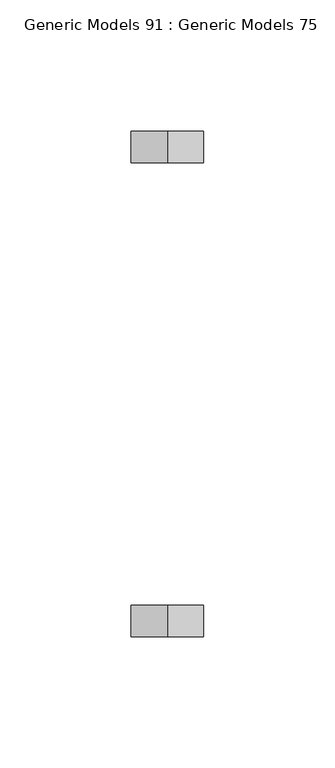
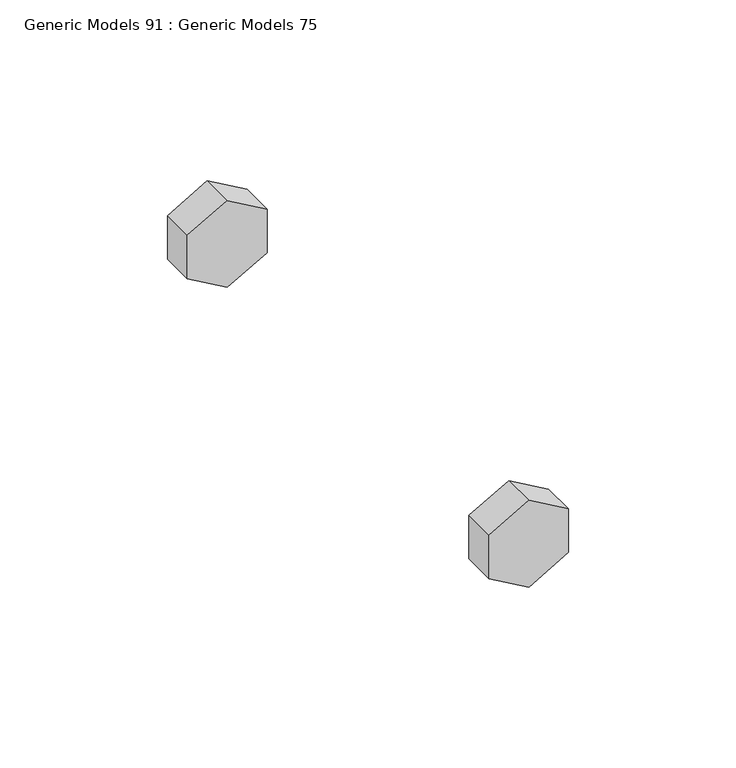
"""IFC4 building model written with IfcOpenShell, lengths in millimetres: proxy geometry, Generic Models 91 : Generic Models 75."""

import ifcopenshell
import ifcopenshell.guid

model = None  # the IFC model being written
_history = None  # IfcOwnerHistory: only IFC2X3 demands one
_inside = {}  # id of a spatial element -> (the spatial element, [elements in it])
_under = {}  # id of a project, library or spatial element -> (it, [spatial elements below it])
_declared = {}  # id of a project -> (the project, [libraries it declares])
_typed = {}  # id of a type object -> (the type object, [elements of that type])
_made_of = {}  # id of a material, layer set ... -> (it, [elements and type objects made of it])


def new_model(schema):
    """Start an empty IFC model of exactly this schema.

    Asked for "IFC4X3", IfcOpenShell would pick the latest addendum, in which some entities
    have other attributes; the version numbers below select the first issue.
    IFC2X3 requires an IfcOwnerHistory on every rooted entity: one is made here for all.
    """
    global model, _history
    if schema == "IFC4X3":
        model = ifcopenshell.file(schema_version=(4, 3, 0, 0))
    else:
        model = ifcopenshell.file(schema=schema)
    _inside.clear()
    _under.clear()
    _declared.clear()
    _typed.clear()
    _made_of.clear()
    _history = None
    if model.schema == "IFC2X3":
        org = make("IfcOrganization", Name="unknown")
        user = make(
            "IfcPersonAndOrganization",
            ThePerson=make("IfcPerson", FamilyName="unknown"),
            TheOrganization=org,
        )
        app = make(
            "IfcApplication",
            ApplicationDeveloper=org,
            Version="unknown",
            ApplicationFullName="unknown",
            ApplicationIdentifier="unknown",
        )
        _history = make(
            "IfcOwnerHistory",
            OwningUser=user,
            OwningApplication=app,
            ChangeAction="ADDED",
            CreationDate=0,
        )
    return model


def make(cls, **values):
    """One entity of the class cls with the attributes given. An attribute that is None is left unset."""
    return model.create_entity(
        cls, **{name: value for name, value in values.items() if value is not None}
    )


def rooted(cls, **values):
    """An entity with a GlobalId (a new one), such as an element, a storey or a relation."""
    return make(cls, GlobalId=ifcopenshell.guid.new(), OwnerHistory=_history, **values)


def si_unit(unit_type, name, prefix=None):
    """IfcSIUnit, for example si_unit("LENGTHUNIT", "METRE", prefix="MILLI")."""
    return make("IfcSIUnit", UnitType=unit_type, Prefix=prefix, Name=name)


def assignment(units):
    """IfcUnitAssignment: the units of a project."""
    return None if units is None else make("IfcUnitAssignment", Units=units)


def point(xyz):
    """IfcCartesianPoint."""
    return None if xyz is None else make("IfcCartesianPoint", Coordinates=xyz)


def direction(xyz):
    """IfcDirection."""
    return None if xyz is None else make("IfcDirection", DirectionRatios=xyz)


def frame(location, z_axis=None, x_axis=None):
    """IfcAxis2Placement3D, a coordinate frame: its origin and axes. An axis left out is left unset."""
    return make(
        "IfcAxis2Placement3D",
        Location=point(location),
        Axis=direction(z_axis),
        RefDirection=direction(x_axis),
    )


def origin():
    """The frame at (0, 0, 0) with its axes left unset."""
    return frame((0.0, 0.0, 0.0))


def place(relative_to, where):
    """IfcLocalPlacement: puts the frame where relative to a parent placement (None: the world)."""
    return make(
        "IfcLocalPlacement", PlacementRelTo=relative_to, RelativePlacement=where
    )


def context(
    kind, dimensions, precision=None, world=None, true_north=None, identifier=None
):
    """IfcGeometricRepresentationContext, for example the 3D "Model" context."""
    return make(
        "IfcGeometricRepresentationContext",
        ContextIdentifier=identifier,
        ContextType=kind,
        CoordinateSpaceDimension=dimensions,
        Precision=precision,
        WorldCoordinateSystem=world,
        TrueNorth=true_north,
    )


def project(units=None, contexts=None):
    """IfcProject with its units and contexts."""
    return rooted(
        "IfcProject",
        Name="project",
        RepresentationContexts=contexts,
        UnitsInContext=assignment(units),
    )


def spatial(cls, under=None, at=None, **own):
    """A site, building, storey or space (cls), placed at a placement, below another one or the project."""
    s = rooted(cls, ObjectPlacement=at, **own)
    if under is not None:
        _under.setdefault(under.id(), (under, []))[1].append(s)
    return s


def polyline(points):
    """IfcPolyline through the points."""
    return make("IfcPolyline", Points=[point(p) for p in points])


def outline(outer, holes=None, kind="AREA"):
    """IfcArbitraryClosedProfileDef: a profile drawn as a closed curve; with holes, ...WithVoids."""
    if holes is None:
        return make("IfcArbitraryClosedProfileDef", ProfileType=kind, OuterCurve=outer)
    return make(
        "IfcArbitraryProfileDefWithVoids",
        ProfileType=kind,
        OuterCurve=outer,
        InnerCurves=holes,
    )


def extrude(swept, where, along, depth):
    """IfcExtrudedAreaSolid: the profile swept, set in the frame where, extruded along a direction by depth."""
    return make(
        "IfcExtrudedAreaSolid",
        SweptArea=swept,
        Position=where,
        ExtrudedDirection=direction(along),
        Depth=depth,
    )


def shape(context_of_items, identifier, shape_type, items):
    """IfcShapeRepresentation: the items that make up one representation, for example the "Body"."""
    return make(
        "IfcShapeRepresentation",
        ContextOfItems=context_of_items,
        RepresentationIdentifier=identifier,
        RepresentationType=shape_type,
        Items=items,
    )


def source(mapping_origin, context_of_items, identifier, shape_type, items):
    """IfcRepresentationMap: a shape defined once, which mapped items show again and again."""
    return make(
        "IfcRepresentationMap",
        MappingOrigin=mapping_origin,
        MappedRepresentation=shape(context_of_items, identifier, shape_type, items),
    )


def transform(
    local_origin,
    x_axis=None,
    y_axis=None,
    z_axis=None,
    scale=None,
    scale2=None,
    scale3=None,
    uniform=True,
):
    """IfcCartesianTransformationOperator3D, or its non-uniform kind. x_axis, y_axis, z_axis: its Axis1, 2, 3."""
    if uniform:
        return make(
            "IfcCartesianTransformationOperator3D",
            Axis1=direction(x_axis),
            Axis2=direction(y_axis),
            LocalOrigin=point(local_origin),
            Scale=scale,
            Axis3=direction(z_axis),
        )
    return make(
        "IfcCartesianTransformationOperator3DnonUniform",
        Axis1=direction(x_axis),
        Axis2=direction(y_axis),
        LocalOrigin=point(local_origin),
        Scale=scale,
        Axis3=direction(z_axis),
        Scale2=scale2,
        Scale3=scale3,
    )


def mapped(mapping_source, mapping_target):
    """IfcMappedItem: shows the shape of a source again, moved by a transform."""
    return make(
        "IfcMappedItem", MappingSource=mapping_source, MappingTarget=mapping_target
    )


def made_of(thing, what):
    """Note that an element or type object is made of a material, layer set ...; save() writes the relation."""
    if what is not None:
        _made_of.setdefault(what.id(), (what, []))[1].append(thing)
    return thing


def element(
    cls,
    number,
    at=None,
    inside=None,
    cuts=None,
    type_object=None,
    material=None,
    context=None,
    identifier="Body",
    shape_type=None,
    held_by="IfcProductDefinitionShape",
    body=None,
    shapes=None,
    **own,
):
    """One element of the class cls, such as IfcWall. Its Tag is "e" and its number.

    at: its placement. inside: the storey or other place that contains it. cuts: it is an
    opening in that element (IfcRelVoidsElement). A single representation is given by context,
    identifier, shape_type and body (its items); several are given by shapes. held_by: the class
    of the entity that holds the representations. save() writes the other relations.
    """
    e = rooted(cls, Tag="e%d" % number, ObjectPlacement=at, **own)
    if body is not None:
        shapes = [shape(context, identifier, shape_type, body)]
    if shapes is not None:
        e.Representation = make(held_by, Representations=shapes)
    if inside is not None:
        _inside.setdefault(inside.id(), (inside, []))[1].append(e)
    if cuts is not None:
        rooted(
            "IfcRelVoidsElement", RelatingBuildingElement=cuts, RelatedOpeningElement=e
        )
    if type_object is not None:
        _typed.setdefault(type_object.id(), (type_object, []))[1].append(e)
    return made_of(e, material)


def aggregate(whole, parts):
    """IfcRelAggregates: a whole, such as a stair, and the parts it consists of."""
    return rooted("IfcRelAggregates", RelatingObject=whole, RelatedObjects=parts)


def save(model, path):
    """Write the relations noted so far, then the file.

    IfcRelAggregates (storeys below a building ...), IfcRelContainedInSpatialStructure (elements
    in a storey), IfcRelDefinesByType, IfcRelAssociatesMaterial and IfcRelDeclares: one each for
    every whole, place, type object, material and project.
    """
    for whole, parts in _under.values():
        aggregate(whole, parts)
    for where, things in _inside.values():
        rooted(
            "IfcRelContainedInSpatialStructure",
            RelatedElements=things,
            RelatingStructure=where,
        )
    for kind, things in _typed.values():
        rooted("IfcRelDefinesByType", RelatedObjects=things, RelatingType=kind)
    for what, things in _made_of.values():
        rooted("IfcRelAssociatesMaterial", RelatedObjects=things, RelatingMaterial=what)
    for by, libraries in _declared.values():
        rooted("IfcRelDeclares", RelatingContext=by, RelatedDefinitions=libraries)
    model.write(path)


def generic_models_91_generic_models_75_28280ab1(model_context):
    return source(origin(), model_context, "Body", "SweptSolid", [
        extrude(outline(polyline([(269298.5462802, 31974.4067029), (269282.7097067, 31974.4067029), (269274.79142, 31988.1215778), (269282.7097067, 32001.8364528), (269298.5462802, 32001.8364528), (269306.464567, 31988.1215778), (269298.5462802, 31974.4067029)])), frame((0.0, 36491.5582942, 0.0), z_axis=(0.0, 1.0, 0.0), x_axis=(0.0, 0.0, 1.0)), (0.0, 0.0, 1.0), 11.90625),
        extrude(outline(polyline([(269298.5462802, 31974.4067029), (269282.7097067, 31974.4067029), (269274.79142, 31988.1215778), (269282.7097067, 32001.8364528), (269298.5462802, 32001.8364528), (269306.464567, 31988.1215778), (269298.5462802, 31974.4067029)])), frame((0.0, 36311.3770442, 0.0), z_axis=(0.0, 1.0, 0.0), x_axis=(0.0, 0.0, 1.0)), (0.0, 0.0, 1.0), 11.90625),
    ])


if __name__ == "__main__":
    model = new_model("IFC4")
    model_context = context("Model", 3, world=origin())
    ifc_project = project(units=[si_unit("LENGTHUNIT", "METRE", prefix="MILLI")], contexts=[model_context])
    site = spatial("IfcSite", under=ifc_project)
    building = spatial("IfcBuilding", under=site)
    placement = place(None, origin())
    generic_models_91_generic_models_75_shape = generic_models_91_generic_models_75_28280ab1(model_context)
    element("IfcBuildingElementProxy", 1, Name="Generic Models 91 : Generic Models 75", ObjectType="Generic Models 91 : Generic Models 75", at=placement, inside=building, context=model_context, shape_type="MappedRepresentation", body=[
        mapped(generic_models_91_generic_models_75_shape, transform((0.0, 0.0, 0.0), x_axis=(1.0, 0.0, 0.0), y_axis=(0.0, 1.0, 0.0), z_axis=(0.0, 0.0, 1.0))),
    ])
    save(model, "model.ifc")

# Revit data of these elements
# Element 1 (IfcBuildingElementProxy, "Generic Models 91 : Generic Models 75")
#   Materials on its faces: "3/4\" GALV. THRU BOLTS"
# Materials
#   "3/4\" GALV. THRU BOLTS": class "Generic", colour RGB 105 69 171, transparency 0, Cost = 0
